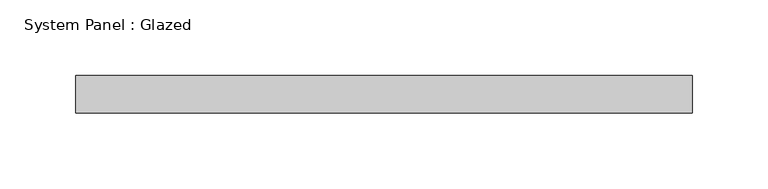
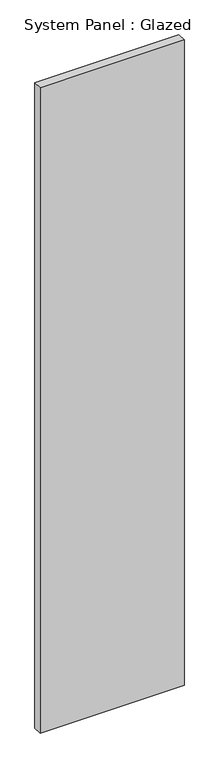
"""IFC4 building model written with IfcOpenShell, lengths in millimetres: plate geometry, System Panel : Glazed."""

from ifc_helpers import new_model, si_unit, origin, origin_with_axes, place, context, project, spatial, polyline, outline, extrude, source, transform, mapped, element, save


def system_panel_glazed_79532cdc(model_context):
    return source(origin(), model_context, "Body", "SweptSolid", [
        extrude(outline(polyline([(204.2039413, 24.5), (-204.2039413, 24.5), (-204.2039413, 49.5), (204.2039413, 49.5), (204.2039413, 24.5)])), origin_with_axes(), (0.0, 0.0, 1.0), 1934.1016494),
    ])


if __name__ == "__main__":
    model = new_model("IFC4")
    model_context = context("Model", 3, world=origin())
    ifc_project = project(units=[si_unit("LENGTHUNIT", "METRE", prefix="MILLI")], contexts=[model_context])
    site = spatial("IfcSite", under=ifc_project)
    building = spatial("IfcBuilding", under=site)
    placement = place(None, origin())
    system_panel_glazed_shape = system_panel_glazed_79532cdc(model_context)
    element("IfcPlate", 1, ObjectType="System Panel : Glazed", at=placement, inside=building, context=model_context, shape_type="MappedRepresentation", body=[
        mapped(system_panel_glazed_shape, transform((0.0, 0.0, 0.0), x_axis=(1.0, 0.0, 0.0), y_axis=(0.0, 1.0, 0.0), z_axis=(0.0, 0.0, 1.0))),
    ])
    save(model, "model.ifc")

# Revit data of these elements
# Type "System Panel : Glazed"
#   Keynote = "H11"
#   Construction Type Id = "GSP4R"
#   Analytic Construction = "1/8 in Pilkington single glazing"
#   Visual Light Transmittance = 0.9
#   Solar Heat Gain Coefficient = 0.86
#   Heat Transfer Coefficient (U) = 6.7069 W/(m²·K)
#   Define Thermal Properties by = 1
# Element 1 (IfcPlate, "System Panel : Glazed")
#   Materials on its faces: "Glass"
# Materials
#   "Glass": class "Glass", colour RGB 0 128 192, transparency 0.9, Description = "Soda Lime Glass", Cost = 0
